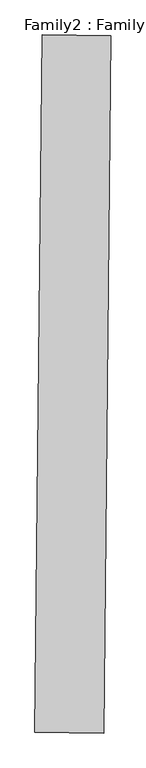
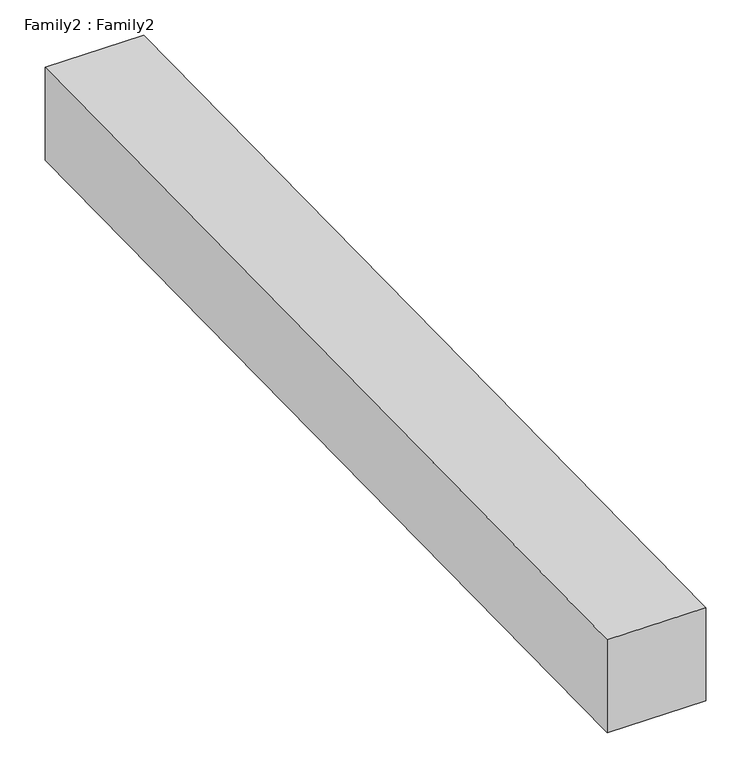
"""IFC4 building model written with IfcOpenShell, lengths in millimetres: proxy geometry, Family2 : Family2."""

import ifcopenshell
import ifcopenshell.guid

model = None  # the IFC model being written
_history = None  # IfcOwnerHistory: only IFC2X3 demands one
_inside = {}  # id of a spatial element -> (the spatial element, [elements in it])
_under = {}  # id of a project, library or spatial element -> (it, [spatial elements below it])
_declared = {}  # id of a project -> (the project, [libraries it declares])
_typed = {}  # id of a type object -> (the type object, [elements of that type])
_made_of = {}  # id of a material, layer set ... -> (it, [elements and type objects made of it])


def new_model(schema):
    """Start an empty IFC model of exactly this schema.

    Asked for "IFC4X3", IfcOpenShell would pick the latest addendum, in which some entities
    have other attributes; the version numbers below select the first issue.
    IFC2X3 requires an IfcOwnerHistory on every rooted entity: one is made here for all.
    """
    global model, _history
    if schema == "IFC4X3":
        model = ifcopenshell.file(schema_version=(4, 3, 0, 0))
    else:
        model = ifcopenshell.file(schema=schema)
    _inside.clear()
    _under.clear()
    _declared.clear()
    _typed.clear()
    _made_of.clear()
    _history = None
    if model.schema == "IFC2X3":
        org = make("IfcOrganization", Name="unknown")
        user = make(
            "IfcPersonAndOrganization",
            ThePerson=make("IfcPerson", FamilyName="unknown"),
            TheOrganization=org,
        )
        app = make(
            "IfcApplication",
            ApplicationDeveloper=org,
            Version="unknown",
            ApplicationFullName="unknown",
            ApplicationIdentifier="unknown",
        )
        _history = make(
            "IfcOwnerHistory",
            OwningUser=user,
            OwningApplication=app,
            ChangeAction="ADDED",
            CreationDate=0,
        )
    return model


def make(cls, **values):
    """One entity of the class cls with the attributes given. An attribute that is None is left unset."""
    return model.create_entity(
        cls, **{name: value for name, value in values.items() if value is not None}
    )


def rooted(cls, **values):
    """An entity with a GlobalId (a new one), such as an element, a storey or a relation."""
    return make(cls, GlobalId=ifcopenshell.guid.new(), OwnerHistory=_history, **values)


def si_unit(unit_type, name, prefix=None):
    """IfcSIUnit, for example si_unit("LENGTHUNIT", "METRE", prefix="MILLI")."""
    return make("IfcSIUnit", UnitType=unit_type, Prefix=prefix, Name=name)


def assignment(units):
    """IfcUnitAssignment: the units of a project."""
    return None if units is None else make("IfcUnitAssignment", Units=units)


def point(xyz):
    """IfcCartesianPoint."""
    return None if xyz is None else make("IfcCartesianPoint", Coordinates=xyz)


def direction(xyz):
    """IfcDirection."""
    return None if xyz is None else make("IfcDirection", DirectionRatios=xyz)


def frame(location, z_axis=None, x_axis=None):
    """IfcAxis2Placement3D, a coordinate frame: its origin and axes. An axis left out is left unset."""
    return make(
        "IfcAxis2Placement3D",
        Location=point(location),
        Axis=direction(z_axis),
        RefDirection=direction(x_axis),
    )


def origin():
    """The frame at (0, 0, 0) with its axes left unset."""
    return frame((0.0, 0.0, 0.0))


def place(relative_to, where):
    """IfcLocalPlacement: puts the frame where relative to a parent placement (None: the world)."""
    return make(
        "IfcLocalPlacement", PlacementRelTo=relative_to, RelativePlacement=where
    )


def context(
    kind, dimensions, precision=None, world=None, true_north=None, identifier=None
):
    """IfcGeometricRepresentationContext, for example the 3D "Model" context."""
    return make(
        "IfcGeometricRepresentationContext",
        ContextIdentifier=identifier,
        ContextType=kind,
        CoordinateSpaceDimension=dimensions,
        Precision=precision,
        WorldCoordinateSystem=world,
        TrueNorth=true_north,
    )


def project(units=None, contexts=None):
    """IfcProject with its units and contexts."""
    return rooted(
        "IfcProject",
        Name="project",
        RepresentationContexts=contexts,
        UnitsInContext=assignment(units),
    )


def spatial(cls, under=None, at=None, **own):
    """A site, building, storey or space (cls), placed at a placement, below another one or the project."""
    s = rooted(cls, ObjectPlacement=at, **own)
    if under is not None:
        _under.setdefault(under.id(), (under, []))[1].append(s)
    return s


def faces_of(points, faces, orient=None, outer=None):
    """IfcFace entities. A face is a list of loops; a loop is a list of indices into points, from 0.

    orient and outer hold one flag for each loop. By default every Orientation is true, the
    first loop of a face is its IfcFaceOuterBound and the others are IfcFaceBound.
    """
    made = []
    for i, loops in enumerate(faces):
        bounds = []
        for j, loop in enumerate(loops):
            is_outer = j == 0 if outer is None else outer[i][j]
            bounds.append(
                make(
                    "IfcFaceOuterBound" if is_outer else "IfcFaceBound",
                    Bound=make("IfcPolyLoop", Polygon=[points[k] for k in loop]),
                    Orientation=True if orient is None else orient[i][j],
                )
            )
        made.append(make("IfcFace", Bounds=bounds))
    return made


def faceted_brep(points, faces, orient=None, outer=None, voids=None):
    """IfcFacetedBrep: a solid bounded by flat faces; with voids (closed shells), ...WithVoids."""
    shared = [point(p) for p in points]
    hull = make("IfcClosedShell", CfsFaces=faces_of(shared, faces, orient, outer))
    if voids is None:
        return make("IfcFacetedBrep", Outer=hull)
    return make(
        "IfcFacetedBrepWithVoids",
        Outer=hull,
        Voids=[
            make(cls, CfsFaces=faces_of(shared, fs, o, b)) for cls, fs, o, b in voids
        ],
    )


def shape(context_of_items, identifier, shape_type, items):
    """IfcShapeRepresentation: the items that make up one representation, for example the "Body"."""
    return make(
        "IfcShapeRepresentation",
        ContextOfItems=context_of_items,
        RepresentationIdentifier=identifier,
        RepresentationType=shape_type,
        Items=items,
    )


def source(mapping_origin, context_of_items, identifier, shape_type, items):
    """IfcRepresentationMap: a shape defined once, which mapped items show again and again."""
    return make(
        "IfcRepresentationMap",
        MappingOrigin=mapping_origin,
        MappedRepresentation=shape(context_of_items, identifier, shape_type, items),
    )


def transform(
    local_origin,
    x_axis=None,
    y_axis=None,
    z_axis=None,
    scale=None,
    scale2=None,
    scale3=None,
    uniform=True,
):
    """IfcCartesianTransformationOperator3D, or its non-uniform kind. x_axis, y_axis, z_axis: its Axis1, 2, 3."""
    if uniform:
        return make(
            "IfcCartesianTransformationOperator3D",
            Axis1=direction(x_axis),
            Axis2=direction(y_axis),
            LocalOrigin=point(local_origin),
            Scale=scale,
            Axis3=direction(z_axis),
        )
    return make(
        "IfcCartesianTransformationOperator3DnonUniform",
        Axis1=direction(x_axis),
        Axis2=direction(y_axis),
        LocalOrigin=point(local_origin),
        Scale=scale,
        Axis3=direction(z_axis),
        Scale2=scale2,
        Scale3=scale3,
    )


def mapped(mapping_source, mapping_target):
    """IfcMappedItem: shows the shape of a source again, moved by a transform."""
    return make(
        "IfcMappedItem", MappingSource=mapping_source, MappingTarget=mapping_target
    )


def made_of(thing, what):
    """Note that an element or type object is made of a material, layer set ...; save() writes the relation."""
    if what is not None:
        _made_of.setdefault(what.id(), (what, []))[1].append(thing)
    return thing


def element(
    cls,
    number,
    at=None,
    inside=None,
    cuts=None,
    type_object=None,
    material=None,
    context=None,
    identifier="Body",
    shape_type=None,
    held_by="IfcProductDefinitionShape",
    body=None,
    shapes=None,
    **own,
):
    """One element of the class cls, such as IfcWall. Its Tag is "e" and its number.

    at: its placement. inside: the storey or other place that contains it. cuts: it is an
    opening in that element (IfcRelVoidsElement). A single representation is given by context,
    identifier, shape_type and body (its items); several are given by shapes. held_by: the class
    of the entity that holds the representations. save() writes the other relations.
    """
    e = rooted(cls, Tag="e%d" % number, ObjectPlacement=at, **own)
    if body is not None:
        shapes = [shape(context, identifier, shape_type, body)]
    if shapes is not None:
        e.Representation = make(held_by, Representations=shapes)
    if inside is not None:
        _inside.setdefault(inside.id(), (inside, []))[1].append(e)
    if cuts is not None:
        rooted(
            "IfcRelVoidsElement", RelatingBuildingElement=cuts, RelatedOpeningElement=e
        )
    if type_object is not None:
        _typed.setdefault(type_object.id(), (type_object, []))[1].append(e)
    return made_of(e, material)


def aggregate(whole, parts):
    """IfcRelAggregates: a whole, such as a stair, and the parts it consists of."""
    return rooted("IfcRelAggregates", RelatingObject=whole, RelatedObjects=parts)


def save(model, path):
    """Write the relations noted so far, then the file.

    IfcRelAggregates (storeys below a building ...), IfcRelContainedInSpatialStructure (elements
    in a storey), IfcRelDefinesByType, IfcRelAssociatesMaterial and IfcRelDeclares: one each for
    every whole, place, type object, material and project.
    """
    for whole, parts in _under.values():
        aggregate(whole, parts)
    for where, things in _inside.values():
        rooted(
            "IfcRelContainedInSpatialStructure",
            RelatedElements=things,
            RelatingStructure=where,
        )
    for kind, things in _typed.values():
        rooted("IfcRelDefinesByType", RelatedObjects=things, RelatingType=kind)
    for what, things in _made_of.values():
        rooted("IfcRelAssociatesMaterial", RelatedObjects=things, RelatingMaterial=what)
    for by, libraries in _declared.values():
        rooted("IfcRelDeclares", RelatingContext=by, RelatedDefinitions=libraries)
    model.write(path)


def family2_family2_a792d820(model_context):
    return source(origin(), model_context, "Body", "Brep", [
        faceted_brep([(-3953.7303514, -7085.2958851, 1.0945136), (-3953.7303514, -7085.2958851, 201.0945136), (-3933.1124431, -5062.3042375, 202.060409), (-3933.1124431, -5062.3042375, 2.060409), (-3753.7391614, -7087.1730977, 201.0945136), (-3733.1212531, -5064.1814502, 202.060409), (-3753.7391614, -7087.1730977, 1.0945136), (-3733.1212531, -5064.1814502, 2.060409)], [[[0, 1, 2, 3]], [[1, 4, 5, 2]], [[4, 6, 7, 5]], [[6, 0, 3, 7]], [[3, 2, 5, 7]], [[0, 6, 4, 1]]]),
    ])


if __name__ == "__main__":
    model = new_model("IFC4")
    model_context = context("Model", 3, world=origin())
    ifc_project = project(units=[si_unit("LENGTHUNIT", "METRE", prefix="MILLI")], contexts=[model_context])
    site = spatial("IfcSite", under=ifc_project)
    building = spatial("IfcBuilding", under=site)
    placement = place(None, origin())
    family2_family2_shape = family2_family2_a792d820(model_context)
    element("IfcBuildingElementProxy", 1, Name="Family2 : Family2", ObjectType="Family2 : Family2", at=placement, inside=building, context=model_context, shape_type="MappedRepresentation", body=[
        mapped(family2_family2_shape, transform((0.0, 0.0, 0.0), x_axis=(1.0, 0.0, 0.0), y_axis=(0.0, 1.0, 0.0), z_axis=(0.0, 0.0, 1.0))),
    ])
    save(model, "model.ifc")

# Revit data of these elements
# Type "Family2 : Family2"
#   Default Elevation = 0
